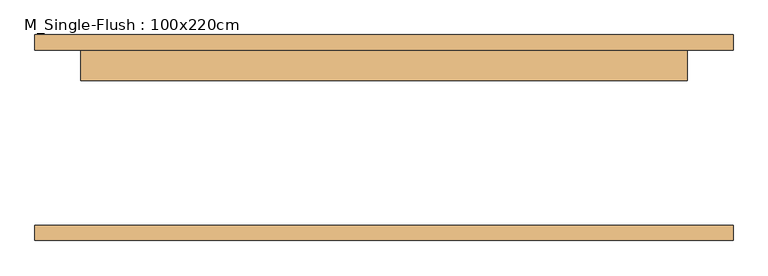
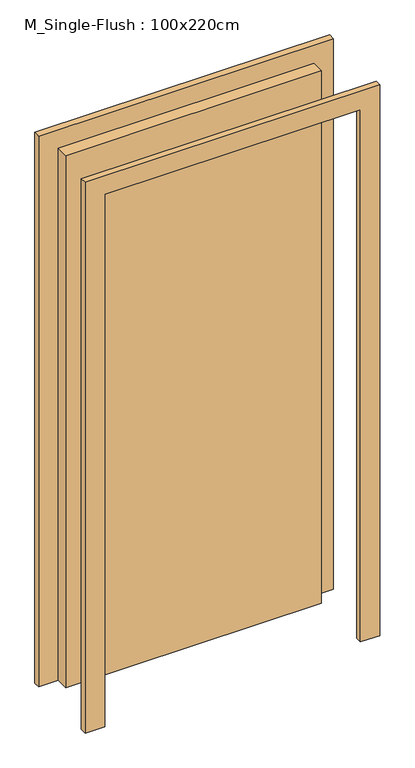
"""IFC4 building model written with IfcOpenShell, lengths in millimetres: door geometry, M_Single-Flush : 100x220cm."""

import ifcopenshell
import ifcopenshell.guid

model = None  # the IFC model being written
_history = None  # IfcOwnerHistory: only IFC2X3 demands one
_inside = {}  # id of a spatial element -> (the spatial element, [elements in it])
_under = {}  # id of a project, library or spatial element -> (it, [spatial elements below it])
_declared = {}  # id of a project -> (the project, [libraries it declares])
_typed = {}  # id of a type object -> (the type object, [elements of that type])
_made_of = {}  # id of a material, layer set ... -> (it, [elements and type objects made of it])


def new_model(schema):
    """Start an empty IFC model of exactly this schema.

    Asked for "IFC4X3", IfcOpenShell would pick the latest addendum, in which some entities
    have other attributes; the version numbers below select the first issue.
    IFC2X3 requires an IfcOwnerHistory on every rooted entity: one is made here for all.
    """
    global model, _history
    if schema == "IFC4X3":
        model = ifcopenshell.file(schema_version=(4, 3, 0, 0))
    else:
        model = ifcopenshell.file(schema=schema)
    _inside.clear()
    _under.clear()
    _declared.clear()
    _typed.clear()
    _made_of.clear()
    _history = None
    if model.schema == "IFC2X3":
        org = make("IfcOrganization", Name="unknown")
        user = make(
            "IfcPersonAndOrganization",
            ThePerson=make("IfcPerson", FamilyName="unknown"),
            TheOrganization=org,
        )
        app = make(
            "IfcApplication",
            ApplicationDeveloper=org,
            Version="unknown",
            ApplicationFullName="unknown",
            ApplicationIdentifier="unknown",
        )
        _history = make(
            "IfcOwnerHistory",
            OwningUser=user,
            OwningApplication=app,
            ChangeAction="ADDED",
            CreationDate=0,
        )
    return model


def make(cls, **values):
    """One entity of the class cls with the attributes given. An attribute that is None is left unset."""
    return model.create_entity(
        cls, **{name: value for name, value in values.items() if value is not None}
    )


def rooted(cls, **values):
    """An entity with a GlobalId (a new one), such as an element, a storey or a relation."""
    return make(cls, GlobalId=ifcopenshell.guid.new(), OwnerHistory=_history, **values)


def si_unit(unit_type, name, prefix=None):
    """IfcSIUnit, for example si_unit("LENGTHUNIT", "METRE", prefix="MILLI")."""
    return make("IfcSIUnit", UnitType=unit_type, Prefix=prefix, Name=name)


def assignment(units):
    """IfcUnitAssignment: the units of a project."""
    return None if units is None else make("IfcUnitAssignment", Units=units)


def point(xyz):
    """IfcCartesianPoint."""
    return None if xyz is None else make("IfcCartesianPoint", Coordinates=xyz)


def direction(xyz):
    """IfcDirection."""
    return None if xyz is None else make("IfcDirection", DirectionRatios=xyz)


def frame(location, z_axis=None, x_axis=None):
    """IfcAxis2Placement3D, a coordinate frame: its origin and axes. An axis left out is left unset."""
    return make(
        "IfcAxis2Placement3D",
        Location=point(location),
        Axis=direction(z_axis),
        RefDirection=direction(x_axis),
    )


def origin():
    """The frame at (0, 0, 0) with its axes left unset."""
    return frame((0.0, 0.0, 0.0))


def origin_with_axes():
    """The frame at (0, 0, 0) with the z axis (0, 0, 1) and the x axis (1, 0, 0) written out."""
    return frame((0.0, 0.0, 0.0), z_axis=(0.0, 0.0, 1.0), x_axis=(1.0, 0.0, 0.0))


def place(relative_to, where):
    """IfcLocalPlacement: puts the frame where relative to a parent placement (None: the world)."""
    return make(
        "IfcLocalPlacement", PlacementRelTo=relative_to, RelativePlacement=where
    )


def context(
    kind, dimensions, precision=None, world=None, true_north=None, identifier=None
):
    """IfcGeometricRepresentationContext, for example the 3D "Model" context."""
    return make(
        "IfcGeometricRepresentationContext",
        ContextIdentifier=identifier,
        ContextType=kind,
        CoordinateSpaceDimension=dimensions,
        Precision=precision,
        WorldCoordinateSystem=world,
        TrueNorth=true_north,
    )


def project(units=None, contexts=None):
    """IfcProject with its units and contexts."""
    return rooted(
        "IfcProject",
        Name="project",
        RepresentationContexts=contexts,
        UnitsInContext=assignment(units),
    )


def spatial(cls, under=None, at=None, **own):
    """A site, building, storey or space (cls), placed at a placement, below another one or the project."""
    s = rooted(cls, ObjectPlacement=at, **own)
    if under is not None:
        _under.setdefault(under.id(), (under, []))[1].append(s)
    return s


def polyline(points):
    """IfcPolyline through the points."""
    return make("IfcPolyline", Points=[point(p) for p in points])


def outline(outer, holes=None, kind="AREA"):
    """IfcArbitraryClosedProfileDef: a profile drawn as a closed curve; with holes, ...WithVoids."""
    if holes is None:
        return make("IfcArbitraryClosedProfileDef", ProfileType=kind, OuterCurve=outer)
    return make(
        "IfcArbitraryProfileDefWithVoids",
        ProfileType=kind,
        OuterCurve=outer,
        InnerCurves=holes,
    )


def extrude(swept, where, along, depth):
    """IfcExtrudedAreaSolid: the profile swept, set in the frame where, extruded along a direction by depth."""
    return make(
        "IfcExtrudedAreaSolid",
        SweptArea=swept,
        Position=where,
        ExtrudedDirection=direction(along),
        Depth=depth,
    )


def shape(context_of_items, identifier, shape_type, items):
    """IfcShapeRepresentation: the items that make up one representation, for example the "Body"."""
    return make(
        "IfcShapeRepresentation",
        ContextOfItems=context_of_items,
        RepresentationIdentifier=identifier,
        RepresentationType=shape_type,
        Items=items,
    )


def source(mapping_origin, context_of_items, identifier, shape_type, items):
    """IfcRepresentationMap: a shape defined once, which mapped items show again and again."""
    return make(
        "IfcRepresentationMap",
        MappingOrigin=mapping_origin,
        MappedRepresentation=shape(context_of_items, identifier, shape_type, items),
    )


def transform(
    local_origin,
    x_axis=None,
    y_axis=None,
    z_axis=None,
    scale=None,
    scale2=None,
    scale3=None,
    uniform=True,
):
    """IfcCartesianTransformationOperator3D, or its non-uniform kind. x_axis, y_axis, z_axis: its Axis1, 2, 3."""
    if uniform:
        return make(
            "IfcCartesianTransformationOperator3D",
            Axis1=direction(x_axis),
            Axis2=direction(y_axis),
            LocalOrigin=point(local_origin),
            Scale=scale,
            Axis3=direction(z_axis),
        )
    return make(
        "IfcCartesianTransformationOperator3DnonUniform",
        Axis1=direction(x_axis),
        Axis2=direction(y_axis),
        LocalOrigin=point(local_origin),
        Scale=scale,
        Axis3=direction(z_axis),
        Scale2=scale2,
        Scale3=scale3,
    )


def mapped(mapping_source, mapping_target):
    """IfcMappedItem: shows the shape of a source again, moved by a transform."""
    return make(
        "IfcMappedItem", MappingSource=mapping_source, MappingTarget=mapping_target
    )


def made_of(thing, what):
    """Note that an element or type object is made of a material, layer set ...; save() writes the relation."""
    if what is not None:
        _made_of.setdefault(what.id(), (what, []))[1].append(thing)
    return thing


def element(
    cls,
    number,
    at=None,
    inside=None,
    cuts=None,
    type_object=None,
    material=None,
    context=None,
    identifier="Body",
    shape_type=None,
    held_by="IfcProductDefinitionShape",
    body=None,
    shapes=None,
    **own,
):
    """One element of the class cls, such as IfcWall. Its Tag is "e" and its number.

    at: its placement. inside: the storey or other place that contains it. cuts: it is an
    opening in that element (IfcRelVoidsElement). A single representation is given by context,
    identifier, shape_type and body (its items); several are given by shapes. held_by: the class
    of the entity that holds the representations. save() writes the other relations.
    """
    e = rooted(cls, Tag="e%d" % number, ObjectPlacement=at, **own)
    if body is not None:
        shapes = [shape(context, identifier, shape_type, body)]
    if shapes is not None:
        e.Representation = make(held_by, Representations=shapes)
    if inside is not None:
        _inside.setdefault(inside.id(), (inside, []))[1].append(e)
    if cuts is not None:
        rooted(
            "IfcRelVoidsElement", RelatingBuildingElement=cuts, RelatedOpeningElement=e
        )
    if type_object is not None:
        _typed.setdefault(type_object.id(), (type_object, []))[1].append(e)
    return made_of(e, material)


def aggregate(whole, parts):
    """IfcRelAggregates: a whole, such as a stair, and the parts it consists of."""
    return rooted("IfcRelAggregates", RelatingObject=whole, RelatedObjects=parts)


def save(model, path):
    """Write the relations noted so far, then the file.

    IfcRelAggregates (storeys below a building ...), IfcRelContainedInSpatialStructure (elements
    in a storey), IfcRelDefinesByType, IfcRelAssociatesMaterial and IfcRelDeclares: one each for
    every whole, place, type object, material and project.
    """
    for whole, parts in _under.values():
        aggregate(whole, parts)
    for where, things in _inside.values():
        rooted(
            "IfcRelContainedInSpatialStructure",
            RelatedElements=things,
            RelatingStructure=where,
        )
    for kind, things in _typed.values():
        rooted("IfcRelDefinesByType", RelatedObjects=things, RelatingType=kind)
    for what, things in _made_of.values():
        rooted("IfcRelAssociatesMaterial", RelatedObjects=things, RelatingMaterial=what)
    for by, libraries in _declared.values():
        rooted("IfcRelDeclares", RelatingContext=by, RelatedDefinitions=libraries)
    model.write(path)


def m_single_flush_100x220cm_28528f9a(model_context):
    return source(origin(), model_context, "Body", "SweptSolid", [
        extrude(outline(polyline([(2276.0, -576.0), (0.0, -576.0), (0.0, -500.0), (2200.0, -500.0), (2200.0, 500.0), (0.0, 500.0), (0.0, 576.0), (2276.0, 576.0), (2276.0, -576.0)])), frame((0.0, 145.0, 0.0), z_axis=(0.0, 1.0, 0.0), x_axis=(0.0, 0.0, 1.0)), (0.0, 0.0, 1.0), 25.0),
        extrude(outline(polyline([(2276.0, 576.0), (2276.0, -576.0), (0.0, -576.0), (0.0, -500.0), (2200.0, -500.0), (2200.0, 500.0), (0.0, 500.0), (0.0, 576.0), (2276.0, 576.0)])), frame((0.0, -170.0, 0.0), z_axis=(0.0, 1.0, 0.0), x_axis=(0.0, 0.0, 1.0)), (0.0, 0.0, 1.0), 25.0),
        extrude(outline(polyline([(500.0, 94.0), (-500.0, 94.0), (-500.0, 145.0), (500.0, 145.0), (500.0, 94.0)])), origin_with_axes(), (0.0, 0.0, 1.0), 2200.0),
    ])


if __name__ == "__main__":
    model = new_model("IFC4")
    model_context = context("Model", 3, world=origin())
    ifc_project = project(units=[si_unit("LENGTHUNIT", "METRE", prefix="MILLI")], contexts=[model_context])
    site = spatial("IfcSite", under=ifc_project)
    building = spatial("IfcBuilding", under=site)
    placement = place(None, origin())
    m_single_flush_100x220cm_shape = m_single_flush_100x220cm_28528f9a(model_context)
    element("IfcDoor", 1, ObjectType="M_Single-Flush : 100x220cm", at=placement, inside=building, context=model_context, shape_type="MappedRepresentation", body=[
        mapped(m_single_flush_100x220cm_shape, transform((0.0, 0.0, 0.0), x_axis=(1.0, 0.0, 0.0), y_axis=(0.0, 1.0, 0.0), z_axis=(0.0, 0.0, 1.0))),
    ])
    save(model, "model.ifc")

# Revit data of these elements
# Type "M_Single-Flush : 100x220cm"
#   Type Mark = "44"
#   Construction Type Id = "MDOOR"
#   Analytic Construction = "Metal"
#   Thickness = 5.10 cm
#   Heat Transfer Coefficient (U) = 3.7021 W/(m²·K)
#   Height = 220.00 cm
#   Trim Projection Ext = 2.50 cm
#   Trim Projection Int = 2.50 cm
#   Trim Width = 7.60 cm
#   Width = 100.00 cm
#   Define Thermal Properties by = 1
#   Door Material = Door - Panel
#   Frame Material = Door - Frame
#   Visual Light Transmittance = 0
#   Solar Heat Gain Coefficient = 0
#   Function = (empty or 0)
#   Wall Closure = (empty or 0)
# Element 1 (IfcDoor, "M_Single-Flush : 100x220cm")
#   Materials on its faces: "Door - Frame", "Door - Panel"
# Materials
#   "Door - Panel": class "Wood", colour RGB 210 159 95, transparency 0, Cost = 0
#   "Door - Frame": class "Miscellaneous", colour RGB 118 70 51, transparency 0, Cost = 0
